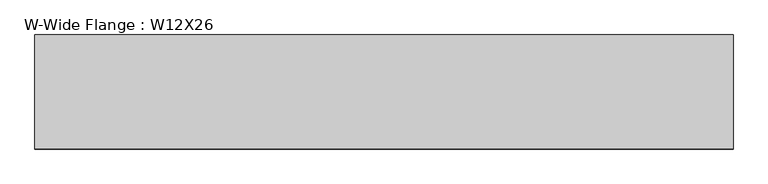
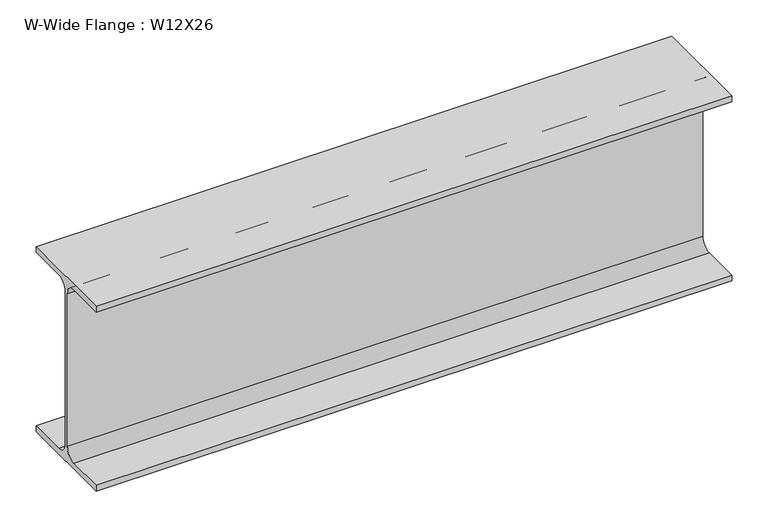
"""IFC4 building model written with IfcOpenShell, lengths in millimetres: beam geometry, W-Wide Flange : W12X26."""

import ifcopenshell
import ifcopenshell.guid

model = None  # the IFC model being written
_history = None  # IfcOwnerHistory: only IFC2X3 demands one
_inside = {}  # id of a spatial element -> (the spatial element, [elements in it])
_under = {}  # id of a project, library or spatial element -> (it, [spatial elements below it])
_declared = {}  # id of a project -> (the project, [libraries it declares])
_typed = {}  # id of a type object -> (the type object, [elements of that type])
_made_of = {}  # id of a material, layer set ... -> (it, [elements and type objects made of it])


def new_model(schema):
    """Start an empty IFC model of exactly this schema.

    Asked for "IFC4X3", IfcOpenShell would pick the latest addendum, in which some entities
    have other attributes; the version numbers below select the first issue.
    IFC2X3 requires an IfcOwnerHistory on every rooted entity: one is made here for all.
    """
    global model, _history
    if schema == "IFC4X3":
        model = ifcopenshell.file(schema_version=(4, 3, 0, 0))
    else:
        model = ifcopenshell.file(schema=schema)
    _inside.clear()
    _under.clear()
    _declared.clear()
    _typed.clear()
    _made_of.clear()
    _history = None
    if model.schema == "IFC2X3":
        org = make("IfcOrganization", Name="unknown")
        user = make(
            "IfcPersonAndOrganization",
            ThePerson=make("IfcPerson", FamilyName="unknown"),
            TheOrganization=org,
        )
        app = make(
            "IfcApplication",
            ApplicationDeveloper=org,
            Version="unknown",
            ApplicationFullName="unknown",
            ApplicationIdentifier="unknown",
        )
        _history = make(
            "IfcOwnerHistory",
            OwningUser=user,
            OwningApplication=app,
            ChangeAction="ADDED",
            CreationDate=0,
        )
    return model


def make(cls, **values):
    """One entity of the class cls with the attributes given. An attribute that is None is left unset."""
    return model.create_entity(
        cls, **{name: value for name, value in values.items() if value is not None}
    )


def rooted(cls, **values):
    """An entity with a GlobalId (a new one), such as an element, a storey or a relation."""
    return make(cls, GlobalId=ifcopenshell.guid.new(), OwnerHistory=_history, **values)


def si_unit(unit_type, name, prefix=None):
    """IfcSIUnit, for example si_unit("LENGTHUNIT", "METRE", prefix="MILLI")."""
    return make("IfcSIUnit", UnitType=unit_type, Prefix=prefix, Name=name)


def assignment(units):
    """IfcUnitAssignment: the units of a project."""
    return None if units is None else make("IfcUnitAssignment", Units=units)


def point(xyz):
    """IfcCartesianPoint."""
    return None if xyz is None else make("IfcCartesianPoint", Coordinates=xyz)


def direction(xyz):
    """IfcDirection."""
    return None if xyz is None else make("IfcDirection", DirectionRatios=xyz)


def frame(location, z_axis=None, x_axis=None):
    """IfcAxis2Placement3D, a coordinate frame: its origin and axes. An axis left out is left unset."""
    return make(
        "IfcAxis2Placement3D",
        Location=point(location),
        Axis=direction(z_axis),
        RefDirection=direction(x_axis),
    )


def frame_2d(location, x_axis=None):
    """IfcAxis2Placement2D, a coordinate frame in the plane: its origin and x axis."""
    return make(
        "IfcAxis2Placement2D", Location=point(location), RefDirection=direction(x_axis)
    )


def origin():
    """The frame at (0, 0, 0) with its axes left unset."""
    return frame((0.0, 0.0, 0.0))


def place(relative_to, where):
    """IfcLocalPlacement: puts the frame where relative to a parent placement (None: the world)."""
    return make(
        "IfcLocalPlacement", PlacementRelTo=relative_to, RelativePlacement=where
    )


def context(
    kind, dimensions, precision=None, world=None, true_north=None, identifier=None
):
    """IfcGeometricRepresentationContext, for example the 3D "Model" context."""
    return make(
        "IfcGeometricRepresentationContext",
        ContextIdentifier=identifier,
        ContextType=kind,
        CoordinateSpaceDimension=dimensions,
        Precision=precision,
        WorldCoordinateSystem=world,
        TrueNorth=true_north,
    )


def project(units=None, contexts=None):
    """IfcProject with its units and contexts."""
    return rooted(
        "IfcProject",
        Name="project",
        RepresentationContexts=contexts,
        UnitsInContext=assignment(units),
    )


def spatial(cls, under=None, at=None, **own):
    """A site, building, storey or space (cls), placed at a placement, below another one or the project."""
    s = rooted(cls, ObjectPlacement=at, **own)
    if under is not None:
        _under.setdefault(under.id(), (under, []))[1].append(s)
    return s


def polyline(points):
    """IfcPolyline through the points."""
    return make("IfcPolyline", Points=[point(p) for p in points])


def circle_curve(where, radius):
    """IfcCircle in the frame where."""
    return make("IfcCircle", Position=where, Radius=radius)


def trimmed(basis, trim1, trim2, sense, master):
    """IfcTrimmedCurve: the piece of a basis curve between two trims."""
    return make(
        "IfcTrimmedCurve",
        BasisCurve=basis,
        Trim1=trim1,
        Trim2=trim2,
        SenseAgreement=sense,
        MasterRepresentation=master,
    )


def segment(curve, same_sense, transition):
    """IfcCompositeCurveSegment."""
    return make(
        "IfcCompositeCurveSegment",
        Transition=transition,
        SameSense=same_sense,
        ParentCurve=curve,
    )


def composite_curve(segments, self_intersect=None):
    """IfcCompositeCurve: segments joined end to end."""
    return make("IfcCompositeCurve", Segments=segments, SelfIntersect=self_intersect)


def outline(outer, holes=None, kind="AREA"):
    """IfcArbitraryClosedProfileDef: a profile drawn as a closed curve; with holes, ...WithVoids."""
    if holes is None:
        return make("IfcArbitraryClosedProfileDef", ProfileType=kind, OuterCurve=outer)
    return make(
        "IfcArbitraryProfileDefWithVoids",
        ProfileType=kind,
        OuterCurve=outer,
        InnerCurves=holes,
    )


def extrude(swept, where, along, depth):
    """IfcExtrudedAreaSolid: the profile swept, set in the frame where, extruded along a direction by depth."""
    return make(
        "IfcExtrudedAreaSolid",
        SweptArea=swept,
        Position=where,
        ExtrudedDirection=direction(along),
        Depth=depth,
    )


def shape(context_of_items, identifier, shape_type, items):
    """IfcShapeRepresentation: the items that make up one representation, for example the "Body"."""
    return make(
        "IfcShapeRepresentation",
        ContextOfItems=context_of_items,
        RepresentationIdentifier=identifier,
        RepresentationType=shape_type,
        Items=items,
    )


def source(mapping_origin, context_of_items, identifier, shape_type, items):
    """IfcRepresentationMap: a shape defined once, which mapped items show again and again."""
    return make(
        "IfcRepresentationMap",
        MappingOrigin=mapping_origin,
        MappedRepresentation=shape(context_of_items, identifier, shape_type, items),
    )


def transform(
    local_origin,
    x_axis=None,
    y_axis=None,
    z_axis=None,
    scale=None,
    scale2=None,
    scale3=None,
    uniform=True,
):
    """IfcCartesianTransformationOperator3D, or its non-uniform kind. x_axis, y_axis, z_axis: its Axis1, 2, 3."""
    if uniform:
        return make(
            "IfcCartesianTransformationOperator3D",
            Axis1=direction(x_axis),
            Axis2=direction(y_axis),
            LocalOrigin=point(local_origin),
            Scale=scale,
            Axis3=direction(z_axis),
        )
    return make(
        "IfcCartesianTransformationOperator3DnonUniform",
        Axis1=direction(x_axis),
        Axis2=direction(y_axis),
        LocalOrigin=point(local_origin),
        Scale=scale,
        Axis3=direction(z_axis),
        Scale2=scale2,
        Scale3=scale3,
    )


def mapped(mapping_source, mapping_target):
    """IfcMappedItem: shows the shape of a source again, moved by a transform."""
    return make(
        "IfcMappedItem", MappingSource=mapping_source, MappingTarget=mapping_target
    )


def made_of(thing, what):
    """Note that an element or type object is made of a material, layer set ...; save() writes the relation."""
    if what is not None:
        _made_of.setdefault(what.id(), (what, []))[1].append(thing)
    return thing


def element(
    cls,
    number,
    at=None,
    inside=None,
    cuts=None,
    type_object=None,
    material=None,
    context=None,
    identifier="Body",
    shape_type=None,
    held_by="IfcProductDefinitionShape",
    body=None,
    shapes=None,
    **own,
):
    """One element of the class cls, such as IfcWall. Its Tag is "e" and its number.

    at: its placement. inside: the storey or other place that contains it. cuts: it is an
    opening in that element (IfcRelVoidsElement). A single representation is given by context,
    identifier, shape_type and body (its items); several are given by shapes. held_by: the class
    of the entity that holds the representations. save() writes the other relations.
    """
    e = rooted(cls, Tag="e%d" % number, ObjectPlacement=at, **own)
    if body is not None:
        shapes = [shape(context, identifier, shape_type, body)]
    if shapes is not None:
        e.Representation = make(held_by, Representations=shapes)
    if inside is not None:
        _inside.setdefault(inside.id(), (inside, []))[1].append(e)
    if cuts is not None:
        rooted(
            "IfcRelVoidsElement", RelatingBuildingElement=cuts, RelatedOpeningElement=e
        )
    if type_object is not None:
        _typed.setdefault(type_object.id(), (type_object, []))[1].append(e)
    return made_of(e, material)


def aggregate(whole, parts):
    """IfcRelAggregates: a whole, such as a stair, and the parts it consists of."""
    return rooted("IfcRelAggregates", RelatingObject=whole, RelatedObjects=parts)


def save(model, path):
    """Write the relations noted so far, then the file.

    IfcRelAggregates (storeys below a building ...), IfcRelContainedInSpatialStructure (elements
    in a storey), IfcRelDefinesByType, IfcRelAssociatesMaterial and IfcRelDeclares: one each for
    every whole, place, type object, material and project.
    """
    for whole, parts in _under.values():
        aggregate(whole, parts)
    for where, things in _inside.values():
        rooted(
            "IfcRelContainedInSpatialStructure",
            RelatedElements=things,
            RelatingStructure=where,
        )
    for kind, things in _typed.values():
        rooted("IfcRelDefinesByType", RelatedObjects=things, RelatingType=kind)
    for what, things in _made_of.values():
        rooted("IfcRelAssociatesMaterial", RelatedObjects=things, RelatingMaterial=what)
    for by, libraries in _declared.values():
        rooted("IfcRelDeclares", RelatingContext=by, RelatedDefinitions=libraries)
    model.write(path)


def w_wide_flange_w12x26_f3e98df9(model_context):
    return source(origin(), model_context, "Body", "SweptSolid", [
        extrude(outline(composite_curve([segment(polyline([(82.4011719, -145.5539063), (82.4011719, -155.178125), (-82.4011719, -155.178125), (-82.4011719, -145.5539063), (-20.2902344, -145.5539063)]), True, "CONTINUOUS"), segment(trimmed(circle_curve(frame_2d((-20.2902344, -128.190625)), 17.3632812), [point((-20.2902344, -145.5539063))], [point((-2.9269531, -128.190625))], True, "CARTESIAN"), True, "CONTINUOUS"), segment(polyline([(-2.9269531, -128.190625), (-2.9269531, 128.190625)]), True, "CONTINUOUS"), segment(trimmed(circle_curve(frame_2d((-20.2902344, 128.190625)), 17.3632812), [point((-2.9269531, 128.190625))], [point((-20.2902344, 145.5539062))], True, "CARTESIAN"), True, "CONTINUOUS"), segment(polyline([(-20.2902344, 145.5539062), (-82.4011719, 145.5539062), (-82.4011719, 155.178125), (82.4011719, 155.178125), (82.4011719, 145.5539062), (20.2902344, 145.5539062)]), True, "CONTINUOUS"), segment(trimmed(circle_curve(frame_2d((20.2902344, 128.190625)), 17.3632812), [point((20.2902344, 145.5539062))], [point((2.9269531, 128.190625))], True, "CARTESIAN"), True, "CONTINUOUS"), segment(polyline([(2.9269531, 128.190625), (2.9269531, -128.190625)]), True, "CONTINUOUS"), segment(trimmed(circle_curve(frame_2d((20.2902344, -128.190625)), 17.3632812), [point((2.9269531, -128.190625))], [point((20.2902344, -145.5539063))], True, "CARTESIAN"), True, "CONTINUOUS"), segment(polyline([(20.2902344, -145.5539063), (82.4011719, -145.5539063)]), True, "CONTINUOUS")], self_intersect=False)), frame((-312.7482318, 0.0, 0.0), z_axis=(1.0, 0.0, 0.0), x_axis=(0.0, 1.0, 0.0)), (0.0, 0.0, 1.0), 1008.7105539),
    ])


if __name__ == "__main__":
    model = new_model("IFC4")
    model_context = context("Model", 3, world=origin())
    ifc_project = project(units=[si_unit("LENGTHUNIT", "METRE", prefix="MILLI")], contexts=[model_context])
    site = spatial("IfcSite", under=ifc_project)
    building = spatial("IfcBuilding", under=site)
    placement = place(None, origin())
    w_wide_flange_w12x26_shape = w_wide_flange_w12x26_f3e98df9(model_context)
    element("IfcBeam", 1, ObjectType="W-Wide Flange : W12X26", at=placement, inside=building, context=model_context, shape_type="MappedRepresentation", body=[
        mapped(w_wide_flange_w12x26_shape, transform((0.0, 0.0, 0.0), x_axis=(1.0, 0.0, 0.0), y_axis=(0.0, 1.0, 0.0), z_axis=(0.0, 0.0, 1.0))),
    ])
    save(model, "model.ifc")

# Revit data of these elements
# Type "W-Wide Flange : W12X26"
#   Assembly Code = "B10"
#   W = 26
#   Length [instance default] = 5' - 0"
#   bf = 0' - 6 125/256"
#   d = 1' - 0 7/32"
#   k = 0' - 1 1/16"
#   k2 = 0' - 0 175/256"
#   tf = 0' - 0 97/256"
#   tw = 0' - 0 59/256"
#   A = 0.053125 SF
#   Structural Material [instance default] = none
# Element 1 (IfcBeam, "W-Wide Flange : W12X26")
#   Structural Material = W 12 X 26
#   Materials on its faces: "W 12 X 26"
# Materials
#   "W 12 X 26": class "Metal", colour RGB 199 199 199, transparency 0, Description = "Carbon steel", Cost = 0
